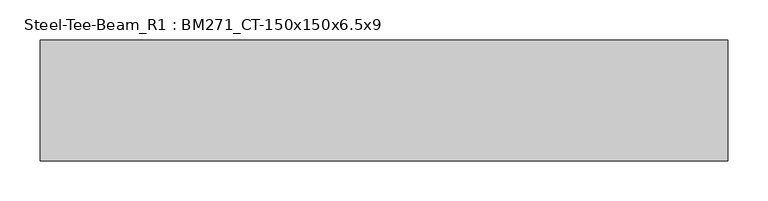
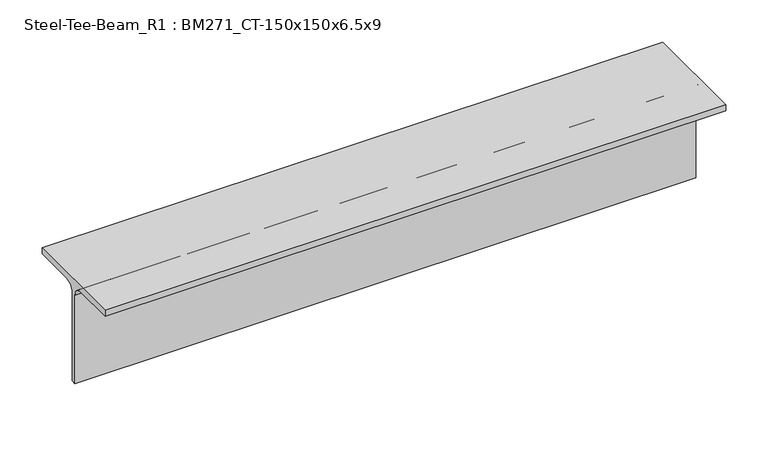
"""IFC4 building model written with IfcOpenShell, lengths in millimetres: member geometry, Steel-Tee-Beam_R1 : BM271_CT-150x150x6.5x9."""

from ifc_helpers import new_model, si_unit, point, frame, frame_2d, origin, place, context, project, spatial, polyline, circle_curve, trimmed, segment, composite_curve, outline, extrude, source, transform, mapped, element, save


def steel_tee_beam_r1_bm271_ct_150x150x6_5x9_e1d70a34(model_context):
    return source(origin(), model_context, "Body", "SweptSolid", [
        extrude(outline(composite_curve([segment(polyline([(-75.0, 75.0), (75.0, 75.0), (75.0, 66.0), (16.25, 66.0)]), True, "CONTINUOUS"), segment(trimmed(circle_curve(frame_2d((16.25, 53.0)), 13.0), [point((16.25, 66.0))], [point((3.25, 53.0))], True, "CARTESIAN"), True, "CONTINUOUS"), segment(polyline([(3.25, 53.0), (3.25, -75.0), (-3.25, -75.0), (-3.25, 53.0)]), True, "CONTINUOUS"), segment(trimmed(circle_curve(frame_2d((-16.25, 53.0)), 13.0), [point((-3.25, 53.0))], [point((-16.25, 66.0))], True, "CARTESIAN"), True, "CONTINUOUS"), segment(polyline([(-16.25, 66.0), (-75.0, 66.0), (-75.0, 75.0)]), True, "CONTINUOUS")], self_intersect=False)), frame((-353.0826681, 0.0, 0.0), z_axis=(1.0, 0.0, 0.0), x_axis=(0.0, 1.0, 0.0)), (0.0, 0.0, 1.0), 853.0826681),
    ])


if __name__ == "__main__":
    model = new_model("IFC4")
    model_context = context("Model", 3, world=origin())
    ifc_project = project(units=[si_unit("LENGTHUNIT", "METRE", prefix="MILLI")], contexts=[model_context])
    site = spatial("IfcSite", under=ifc_project)
    building = spatial("IfcBuilding", under=site)
    placement = place(None, origin())
    steel_tee_beam_r1_bm271_ct_150x150x6_5x9_shape = steel_tee_beam_r1_bm271_ct_150x150x6_5x9_e1d70a34(model_context)
    element("IfcMember", 1, ObjectType="Steel-Tee-Beam_R1 : BM271_CT-150x150x6.5x9", at=placement, inside=building, context=model_context, shape_type="MappedRepresentation", body=[
        mapped(steel_tee_beam_r1_bm271_ct_150x150x6_5x9_shape, transform((0.0, 0.0, 0.0), x_axis=(1.0, 0.0, 0.0), y_axis=(0.0, 1.0, 0.0), z_axis=(0.0, 0.0, 1.0))),
    ])
    save(model, "model.ifc")

# Revit data of these elements
# Type "Steel-Tee-Beam_R1 : BM271_CT-150x150x6.5x9"
#   Keynote = "CT-150x150x6.5x9"
#   Surface Area = 0.588841 m²/m
#   Section Area = 23.3904 cm²
#   Mass per Unit Length = 18.3614 kg/m
#   Length [instance default] = 1.5240 m
#   bf = 0.1500 m
#   d = 0.1500 m
#   k = 0.0220 m
#   r = 0.0130 m
#   tf = 0.0090 m
#   tw = 0.0065 m
#   hec_material4 [instance default] = none
#   hec_material3 [instance default] = none
#   hec_material2 [instance default] = none
#   hec_material1 [instance default] = none
#   Structural Material [instance default] = Steel, 45-345
#   Assembly Code = ""
# Element 1 (IfcMember, "Steel-Tee-Beam_R1 : BM271_CT-150x150x6.5x9")
#   Structural Material = none
# Materials
#   "Steel, 45-345": class "Metal", colour RGB 189 187 185, transparency 0, Description = "Steel 345 MPa", Cost = 0
